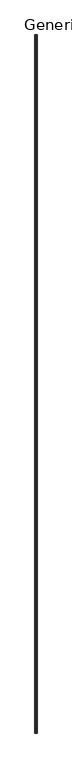
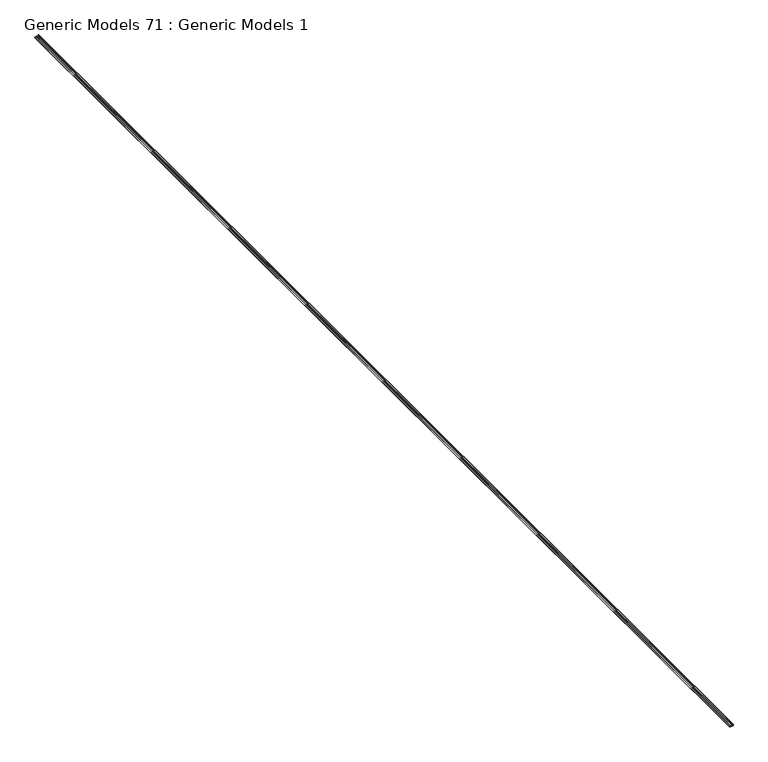
"""IFC4 building model written with IfcOpenShell, lengths in millimetres: proxy geometry, Generic Models 71 : Generic Models 1."""

import ifcopenshell
import ifcopenshell.guid

model = None  # the IFC model being written
_history = None  # IfcOwnerHistory: only IFC2X3 demands one
_inside = {}  # id of a spatial element -> (the spatial element, [elements in it])
_under = {}  # id of a project, library or spatial element -> (it, [spatial elements below it])
_declared = {}  # id of a project -> (the project, [libraries it declares])
_typed = {}  # id of a type object -> (the type object, [elements of that type])
_made_of = {}  # id of a material, layer set ... -> (it, [elements and type objects made of it])


def new_model(schema):
    """Start an empty IFC model of exactly this schema.

    Asked for "IFC4X3", IfcOpenShell would pick the latest addendum, in which some entities
    have other attributes; the version numbers below select the first issue.
    IFC2X3 requires an IfcOwnerHistory on every rooted entity: one is made here for all.
    """
    global model, _history
    if schema == "IFC4X3":
        model = ifcopenshell.file(schema_version=(4, 3, 0, 0))
    else:
        model = ifcopenshell.file(schema=schema)
    _inside.clear()
    _under.clear()
    _declared.clear()
    _typed.clear()
    _made_of.clear()
    _history = None
    if model.schema == "IFC2X3":
        org = make("IfcOrganization", Name="unknown")
        user = make(
            "IfcPersonAndOrganization",
            ThePerson=make("IfcPerson", FamilyName="unknown"),
            TheOrganization=org,
        )
        app = make(
            "IfcApplication",
            ApplicationDeveloper=org,
            Version="unknown",
            ApplicationFullName="unknown",
            ApplicationIdentifier="unknown",
        )
        _history = make(
            "IfcOwnerHistory",
            OwningUser=user,
            OwningApplication=app,
            ChangeAction="ADDED",
            CreationDate=0,
        )
    return model


def make(cls, **values):
    """One entity of the class cls with the attributes given. An attribute that is None is left unset."""
    return model.create_entity(
        cls, **{name: value for name, value in values.items() if value is not None}
    )


def rooted(cls, **values):
    """An entity with a GlobalId (a new one), such as an element, a storey or a relation."""
    return make(cls, GlobalId=ifcopenshell.guid.new(), OwnerHistory=_history, **values)


def si_unit(unit_type, name, prefix=None):
    """IfcSIUnit, for example si_unit("LENGTHUNIT", "METRE", prefix="MILLI")."""
    return make("IfcSIUnit", UnitType=unit_type, Prefix=prefix, Name=name)


def assignment(units):
    """IfcUnitAssignment: the units of a project."""
    return None if units is None else make("IfcUnitAssignment", Units=units)


def point(xyz):
    """IfcCartesianPoint."""
    return None if xyz is None else make("IfcCartesianPoint", Coordinates=xyz)


def direction(xyz):
    """IfcDirection."""
    return None if xyz is None else make("IfcDirection", DirectionRatios=xyz)


def frame(location, z_axis=None, x_axis=None):
    """IfcAxis2Placement3D, a coordinate frame: its origin and axes. An axis left out is left unset."""
    return make(
        "IfcAxis2Placement3D",
        Location=point(location),
        Axis=direction(z_axis),
        RefDirection=direction(x_axis),
    )


def origin():
    """The frame at (0, 0, 0) with its axes left unset."""
    return frame((0.0, 0.0, 0.0))


def place(relative_to, where):
    """IfcLocalPlacement: puts the frame where relative to a parent placement (None: the world)."""
    return make(
        "IfcLocalPlacement", PlacementRelTo=relative_to, RelativePlacement=where
    )


def context(
    kind, dimensions, precision=None, world=None, true_north=None, identifier=None
):
    """IfcGeometricRepresentationContext, for example the 3D "Model" context."""
    return make(
        "IfcGeometricRepresentationContext",
        ContextIdentifier=identifier,
        ContextType=kind,
        CoordinateSpaceDimension=dimensions,
        Precision=precision,
        WorldCoordinateSystem=world,
        TrueNorth=true_north,
    )


def project(units=None, contexts=None):
    """IfcProject with its units and contexts."""
    return rooted(
        "IfcProject",
        Name="project",
        RepresentationContexts=contexts,
        UnitsInContext=assignment(units),
    )


def spatial(cls, under=None, at=None, **own):
    """A site, building, storey or space (cls), placed at a placement, below another one or the project."""
    s = rooted(cls, ObjectPlacement=at, **own)
    if under is not None:
        _under.setdefault(under.id(), (under, []))[1].append(s)
    return s


def polyline(points):
    """IfcPolyline through the points."""
    return make("IfcPolyline", Points=[point(p) for p in points])


def outline(outer, holes=None, kind="AREA"):
    """IfcArbitraryClosedProfileDef: a profile drawn as a closed curve; with holes, ...WithVoids."""
    if holes is None:
        return make("IfcArbitraryClosedProfileDef", ProfileType=kind, OuterCurve=outer)
    return make(
        "IfcArbitraryProfileDefWithVoids",
        ProfileType=kind,
        OuterCurve=outer,
        InnerCurves=holes,
    )


def extrude(swept, where, along, depth):
    """IfcExtrudedAreaSolid: the profile swept, set in the frame where, extruded along a direction by depth."""
    return make(
        "IfcExtrudedAreaSolid",
        SweptArea=swept,
        Position=where,
        ExtrudedDirection=direction(along),
        Depth=depth,
    )


def shape(context_of_items, identifier, shape_type, items):
    """IfcShapeRepresentation: the items that make up one representation, for example the "Body"."""
    return make(
        "IfcShapeRepresentation",
        ContextOfItems=context_of_items,
        RepresentationIdentifier=identifier,
        RepresentationType=shape_type,
        Items=items,
    )


def source(mapping_origin, context_of_items, identifier, shape_type, items):
    """IfcRepresentationMap: a shape defined once, which mapped items show again and again."""
    return make(
        "IfcRepresentationMap",
        MappingOrigin=mapping_origin,
        MappedRepresentation=shape(context_of_items, identifier, shape_type, items),
    )


def transform(
    local_origin,
    x_axis=None,
    y_axis=None,
    z_axis=None,
    scale=None,
    scale2=None,
    scale3=None,
    uniform=True,
):
    """IfcCartesianTransformationOperator3D, or its non-uniform kind. x_axis, y_axis, z_axis: its Axis1, 2, 3."""
    if uniform:
        return make(
            "IfcCartesianTransformationOperator3D",
            Axis1=direction(x_axis),
            Axis2=direction(y_axis),
            LocalOrigin=point(local_origin),
            Scale=scale,
            Axis3=direction(z_axis),
        )
    return make(
        "IfcCartesianTransformationOperator3DnonUniform",
        Axis1=direction(x_axis),
        Axis2=direction(y_axis),
        LocalOrigin=point(local_origin),
        Scale=scale,
        Axis3=direction(z_axis),
        Scale2=scale2,
        Scale3=scale3,
    )


def mapped(mapping_source, mapping_target):
    """IfcMappedItem: shows the shape of a source again, moved by a transform."""
    return make(
        "IfcMappedItem", MappingSource=mapping_source, MappingTarget=mapping_target
    )


def made_of(thing, what):
    """Note that an element or type object is made of a material, layer set ...; save() writes the relation."""
    if what is not None:
        _made_of.setdefault(what.id(), (what, []))[1].append(thing)
    return thing


def element(
    cls,
    number,
    at=None,
    inside=None,
    cuts=None,
    type_object=None,
    material=None,
    context=None,
    identifier="Body",
    shape_type=None,
    held_by="IfcProductDefinitionShape",
    body=None,
    shapes=None,
    **own,
):
    """One element of the class cls, such as IfcWall. Its Tag is "e" and its number.

    at: its placement. inside: the storey or other place that contains it. cuts: it is an
    opening in that element (IfcRelVoidsElement). A single representation is given by context,
    identifier, shape_type and body (its items); several are given by shapes. held_by: the class
    of the entity that holds the representations. save() writes the other relations.
    """
    e = rooted(cls, Tag="e%d" % number, ObjectPlacement=at, **own)
    if body is not None:
        shapes = [shape(context, identifier, shape_type, body)]
    if shapes is not None:
        e.Representation = make(held_by, Representations=shapes)
    if inside is not None:
        _inside.setdefault(inside.id(), (inside, []))[1].append(e)
    if cuts is not None:
        rooted(
            "IfcRelVoidsElement", RelatingBuildingElement=cuts, RelatedOpeningElement=e
        )
    if type_object is not None:
        _typed.setdefault(type_object.id(), (type_object, []))[1].append(e)
    return made_of(e, material)


def aggregate(whole, parts):
    """IfcRelAggregates: a whole, such as a stair, and the parts it consists of."""
    return rooted("IfcRelAggregates", RelatingObject=whole, RelatedObjects=parts)


def save(model, path):
    """Write the relations noted so far, then the file.

    IfcRelAggregates (storeys below a building ...), IfcRelContainedInSpatialStructure (elements
    in a storey), IfcRelDefinesByType, IfcRelAssociatesMaterial and IfcRelDeclares: one each for
    every whole, place, type object, material and project.
    """
    for whole, parts in _under.values():
        aggregate(whole, parts)
    for where, things in _inside.values():
        rooted(
            "IfcRelContainedInSpatialStructure",
            RelatedElements=things,
            RelatingStructure=where,
        )
    for kind, things in _typed.values():
        rooted("IfcRelDefinesByType", RelatedObjects=things, RelatingType=kind)
    for what, things in _made_of.values():
        rooted("IfcRelAssociatesMaterial", RelatedObjects=things, RelatingMaterial=what)
    for by, libraries in _declared.values():
        rooted("IfcRelDeclares", RelatingContext=by, RelatedDefinitions=libraries)
    model.write(path)


def generic_models_71_generic_models_1_deb8e508(model_context):
    return source(origin(), model_context, "Body", "SweptSolid", [
        extrude(outline(polyline([(142822.070303, -9211.2597887), (142822.070303, -9230.9447887), (142833.500303, -9230.9447887), (142833.500303, -9246.1847887), (142822.070303, -9246.1847887), (142822.070303, -9268.6279726), (142820.800303, -9268.6279726), (142820.800303, -9244.9147887), (142832.230303, -9244.9147887), (142832.230303, -9232.2147887), (142820.800303, -9232.2147887), (142820.800303, -9209.9897887), (142825.550103, -9209.9897887), (142825.550103, -9210.8486296), (142844.5946817, -9210.8486296), (142844.5946817, -9212.1186296), (142824.280103, -9212.1186296), (142824.280103, -9211.2597887), (142822.070303, -9211.2597887)])), frame((0.0, -7068.1230338, 0.0), z_axis=(0.0, 1.0, 0.0), x_axis=(0.0, 0.0, 1.0)), (0.0, 0.0, 1.0), 19050.0),
    ])


if __name__ == "__main__":
    model = new_model("IFC4")
    model_context = context("Model", 3, world=origin())
    ifc_project = project(units=[si_unit("LENGTHUNIT", "METRE", prefix="MILLI")], contexts=[model_context])
    site = spatial("IfcSite", under=ifc_project)
    building = spatial("IfcBuilding", under=site)
    placement = place(None, origin())
    generic_models_71_generic_models_1_shape = generic_models_71_generic_models_1_deb8e508(model_context)
    element("IfcBuildingElementProxy", 1, Name="Generic Models 71 : Generic Models 1", ObjectType="Generic Models 71 : Generic Models 1", at=placement, inside=building, context=model_context, shape_type="MappedRepresentation", body=[
        mapped(generic_models_71_generic_models_1_shape, transform((0.0, 0.0, 0.0), x_axis=(1.0, 0.0, 0.0), y_axis=(0.0, 1.0, 0.0), z_axis=(0.0, 0.0, 1.0))),
    ])
    save(model, "model.ifc")

# Revit data of these elements
# Element 1 (IfcBuildingElementProxy, "Generic Models 71 : Generic Models 1")
#   Materials on its faces: "_16 GA. COPPER VENTED SOFFIT DRIP SCREED"
# Materials
#   "_16 GA. COPPER VENTED SOFFIT DRIP SCREED": class "Generic", colour RGB 253 192 103, transparency 0, Cost = 0
